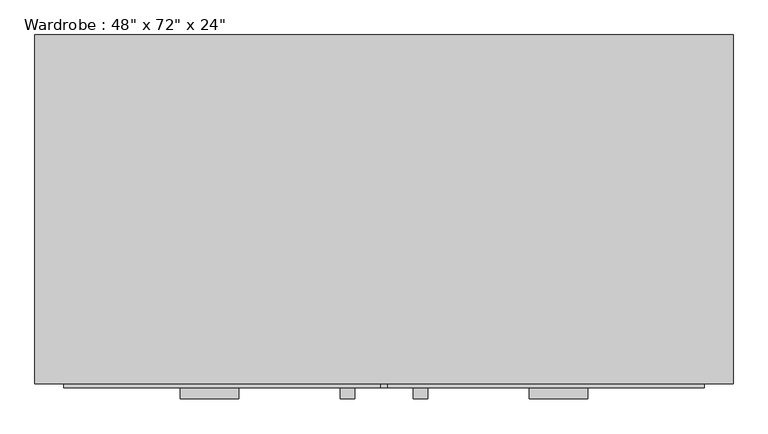
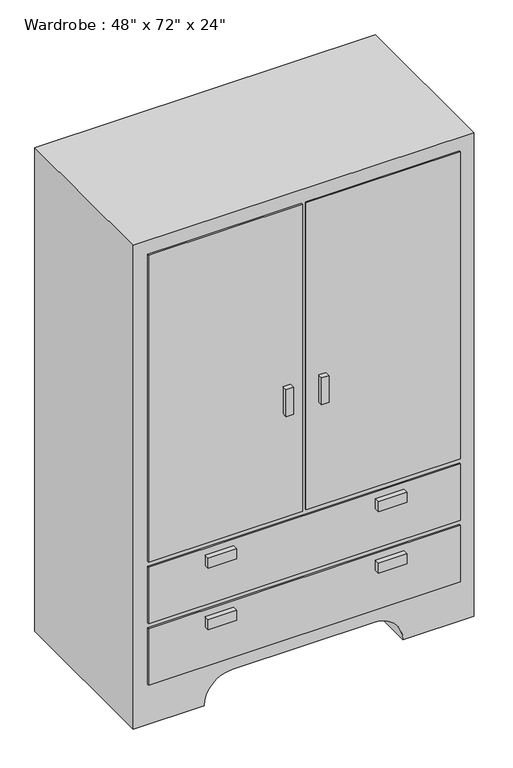
"""IFC4 building model written with IfcOpenShell, lengths in millimetres: furniture geometry."""

from ifc_helpers import new_model, si_unit, point, frame, frame_2d, origin, place, context, project, spatial, polyline, circle_curve, trimmed, segment, composite_curve, outline, extrude, source, transform, mapped, element, save


def furniture_1d34d0b1(model_context):
    return source(origin(), model_context, "Body", "SweptSolid", [
        extrude(outline(composite_curve([segment(polyline([(0.0, 340.4067402), (1828.8, 340.4067402), (1828.8, -878.7932598), (0.0, -878.7932598), (0.0, -624.7932598)]), True, "CONTINUOUS"), segment(trimmed(circle_curve(frame_2d((0.0, -523.1932598)), 101.6), [point((0.0, -624.7932598))], [point((101.6, -523.1932598))], True, "CARTESIAN"), True, "CONTINUOUS"), segment(polyline([(101.6, -523.1932598), (101.6, -15.1932598)]), True, "CONTINUOUS"), segment(trimmed(circle_curve(frame_2d((0.0, -15.1932598)), 101.6), [point((101.6, -15.1932598))], [point((0.0, 86.4067402))], True, "CARTESIAN"), True, "CONTINUOUS"), segment(polyline([(0.0, 86.4067402), (0.0, 340.4067402)]), True, "CONTINUOUS")], self_intersect=False)), frame((0.0, -888.5388096, 0.0), z_axis=(0.0, 1.0, 0.0), x_axis=(0.0, 0.0, 1.0)), (0.0, 0.0, 1.0), 609.6),
        extrude(outline(polyline([(-319.9932598, -913.9388096), (-345.3932598, -913.9388096), (-345.3932598, -894.8888096), (-319.9932598, -894.8888096), (-319.9932598, -913.9388096)])), frame((0.0, 0.0, 1010.5571429), z_axis=(0.0, 0.0, 1.0), x_axis=(1.0, 0.0, 0.0)), (0.0, 0.0, 1.0), 101.6),
        extrude(outline(polyline([(-192.9932598, -913.9388096), (-218.3932598, -913.9388096), (-218.3932598, -894.8888096), (-192.9932598, -894.8888096), (-192.9932598, -913.9388096)])), frame((0.0, 0.0, 1010.5571429), z_axis=(0.0, 0.0, 1.0), x_axis=(1.0, 0.0, 0.0)), (0.0, 0.0, 1.0), 101.6),
        extrude(outline(polyline([(-523.1932598, -913.9388096), (-624.7932598, -913.9388096), (-624.7932598, -894.8888096), (-523.1932598, -894.8888096), (-523.1932598, -913.9388096)])), frame((0.0, 0.0, 534.3071429), z_axis=(0.0, 0.0, 1.0), x_axis=(1.0, 0.0, 0.0)), (0.0, 0.0, 1.0), 38.1),
        extrude(outline(polyline([(86.4067402, -913.9388096), (-15.1932598, -913.9388096), (-15.1932598, -894.8888096), (86.4067402, -894.8888096), (86.4067402, -913.9388096)])), frame((0.0, 0.0, 534.3071429), z_axis=(0.0, 0.0, 1.0), x_axis=(1.0, 0.0, 0.0)), (0.0, 0.0, 1.0), 38.1),
        extrude(outline(polyline([(86.4067402, -913.9388096), (-15.1932598, -913.9388096), (-15.1932598, -894.8888096), (86.4067402, -894.8888096), (86.4067402, -913.9388096)])), frame((0.0, 0.0, 302.0785714), z_axis=(0.0, 0.0, 1.0), x_axis=(1.0, 0.0, 0.0)), (0.0, 0.0, 1.0), 38.1),
        extrude(outline(polyline([(-523.1932598, -913.9388096), (-624.7932598, -913.9388096), (-624.7932598, -894.8888096), (-523.1932598, -894.8888096), (-523.1932598, -913.9388096)])), frame((0.0, 0.0, 302.0785714), z_axis=(0.0, 0.0, 1.0), x_axis=(1.0, 0.0, 0.0)), (0.0, 0.0, 1.0), 38.1),
        extrude(outline(polyline([(289.6067402, -894.8888096), (-827.9932598, -894.8888096), (-827.9932598, -888.5388096), (289.6067402, -888.5388096), (289.6067402, -894.8888096)])), frame((0.0, 0.0, 384.6285714), z_axis=(0.0, 0.0, 1.0), x_axis=(1.0, 0.0, 0.0)), (0.0, 0.0, 1.0), 213.1785714),
        extrude(outline(polyline([(289.6067402, -894.8888096), (-827.9932598, -894.8888096), (-827.9932598, -888.5388096), (289.6067402, -888.5388096), (289.6067402, -894.8888096)])), frame((0.0, 0.0, 152.4), z_axis=(0.0, 0.0, 1.0), x_axis=(1.0, 0.0, 0.0)), (0.0, 0.0, 1.0), 213.1785714),
        extrude(outline(polyline([(-275.5432598, -894.8888096), (-827.9932598, -894.8888096), (-827.9932598, -888.5388096), (-275.5432598, -888.5388096), (-275.5432598, -894.8888096)])), frame((0.0, 0.0, 616.8571429), z_axis=(0.0, 0.0, 1.0), x_axis=(1.0, 0.0, 0.0)), (0.0, 0.0, 1.0), 1161.1428571),
        extrude(outline(polyline([(289.6067402, -894.8888096), (-262.8432598, -894.8888096), (-262.8432598, -888.5388096), (289.6067402, -888.5388096), (289.6067402, -894.8888096)])), frame((0.0, 0.0, 616.8571429), z_axis=(0.0, 0.0, 1.0), x_axis=(1.0, 0.0, 0.0)), (0.0, 0.0, 1.0), 1161.1428571),
    ])


if __name__ == "__main__":
    model = new_model("IFC4")
    model_context = context("Model", 3, world=origin())
    ifc_project = project(units=[si_unit("LENGTHUNIT", "METRE", prefix="MILLI")], contexts=[model_context])
    site = spatial("IfcSite", under=ifc_project)
    building = spatial("IfcBuilding", under=site)
    placement = place(None, origin())
    furniture_shape = furniture_1d34d0b1(model_context)
    element("IfcFurniture", 1, ObjectType="Wardrobe : 48\" x 72\" x 24\"", at=placement, inside=building, context=model_context, shape_type="MappedRepresentation", body=[
        mapped(furniture_shape, transform((0.0, 0.0, 0.0), x_axis=(1.0, 0.0, 0.0), y_axis=(0.0, 1.0, 0.0), z_axis=(0.0, 0.0, 1.0))),
    ])
    save(model, "model.ifc")

# Revit data of these elements
# Type "Wardrobe : 48\" x 72\" x 24\""
#   Model = "Entertainment Center"
#   Manufacturer = "Acme Funriture"
#   Assembly Code = "E2020200"
#   Depth = 2' - 0"
#   Height = 6' - 0"
#   Width = 4' - 0"
#   Material = Birch
#   Default Elevation = 0
# Element 1 (IfcFurniture, "Wardrobe : 48\" x 72\" x 24\"")
#   Materials on its faces: "Birch"
# Materials
#   "Birch": class "Wood", colour RGB 172 132 95, transparency 0, Description = "Betula Alleghaniensis", Cost = 0
